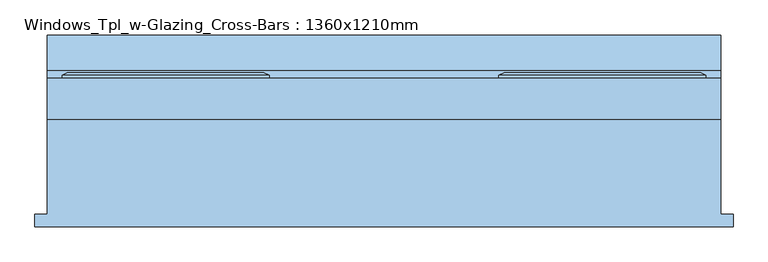
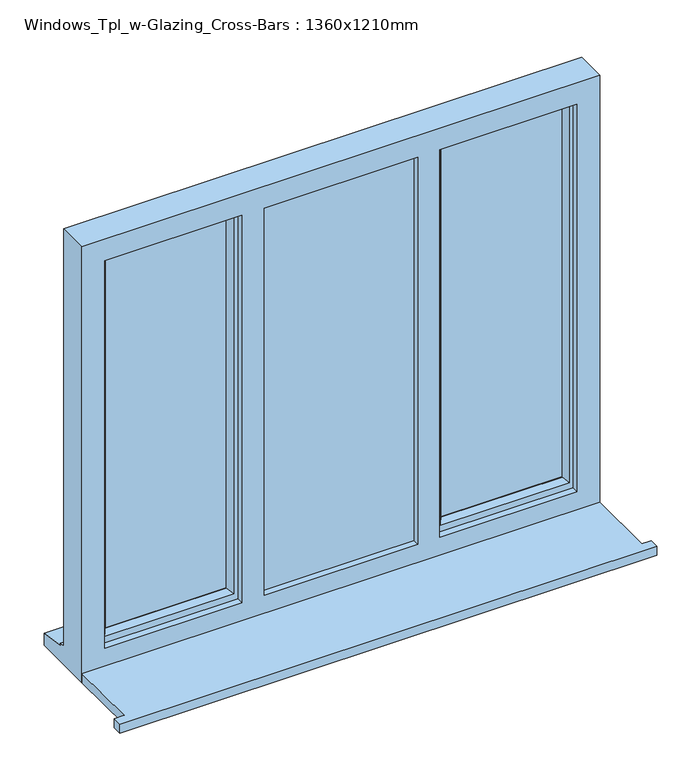
"""IFC4 building model written with IfcOpenShell, lengths in millimetres: window geometry, Windows_Tpl_w-Glazing_Cross-Bars : 1360x1210mm."""

import ifcopenshell
import ifcopenshell.guid

model = None  # the IFC model being written
_history = None  # IfcOwnerHistory: only IFC2X3 demands one
_inside = {}  # id of a spatial element -> (the spatial element, [elements in it])
_under = {}  # id of a project, library or spatial element -> (it, [spatial elements below it])
_declared = {}  # id of a project -> (the project, [libraries it declares])
_typed = {}  # id of a type object -> (the type object, [elements of that type])
_made_of = {}  # id of a material, layer set ... -> (it, [elements and type objects made of it])


def new_model(schema):
    """Start an empty IFC model of exactly this schema.

    Asked for "IFC4X3", IfcOpenShell would pick the latest addendum, in which some entities
    have other attributes; the version numbers below select the first issue.
    IFC2X3 requires an IfcOwnerHistory on every rooted entity: one is made here for all.
    """
    global model, _history
    if schema == "IFC4X3":
        model = ifcopenshell.file(schema_version=(4, 3, 0, 0))
    else:
        model = ifcopenshell.file(schema=schema)
    _inside.clear()
    _under.clear()
    _declared.clear()
    _typed.clear()
    _made_of.clear()
    _history = None
    if model.schema == "IFC2X3":
        org = make("IfcOrganization", Name="unknown")
        user = make(
            "IfcPersonAndOrganization",
            ThePerson=make("IfcPerson", FamilyName="unknown"),
            TheOrganization=org,
        )
        app = make(
            "IfcApplication",
            ApplicationDeveloper=org,
            Version="unknown",
            ApplicationFullName="unknown",
            ApplicationIdentifier="unknown",
        )
        _history = make(
            "IfcOwnerHistory",
            OwningUser=user,
            OwningApplication=app,
            ChangeAction="ADDED",
            CreationDate=0,
        )
    return model


def make(cls, **values):
    """One entity of the class cls with the attributes given. An attribute that is None is left unset."""
    return model.create_entity(
        cls, **{name: value for name, value in values.items() if value is not None}
    )


def rooted(cls, **values):
    """An entity with a GlobalId (a new one), such as an element, a storey or a relation."""
    return make(cls, GlobalId=ifcopenshell.guid.new(), OwnerHistory=_history, **values)


def si_unit(unit_type, name, prefix=None):
    """IfcSIUnit, for example si_unit("LENGTHUNIT", "METRE", prefix="MILLI")."""
    return make("IfcSIUnit", UnitType=unit_type, Prefix=prefix, Name=name)


def assignment(units):
    """IfcUnitAssignment: the units of a project."""
    return None if units is None else make("IfcUnitAssignment", Units=units)


def point(xyz):
    """IfcCartesianPoint."""
    return None if xyz is None else make("IfcCartesianPoint", Coordinates=xyz)


def direction(xyz):
    """IfcDirection."""
    return None if xyz is None else make("IfcDirection", DirectionRatios=xyz)


def frame(location, z_axis=None, x_axis=None):
    """IfcAxis2Placement3D, a coordinate frame: its origin and axes. An axis left out is left unset."""
    return make(
        "IfcAxis2Placement3D",
        Location=point(location),
        Axis=direction(z_axis),
        RefDirection=direction(x_axis),
    )


def origin():
    """The frame at (0, 0, 0) with its axes left unset."""
    return frame((0.0, 0.0, 0.0))


def place(relative_to, where):
    """IfcLocalPlacement: puts the frame where relative to a parent placement (None: the world)."""
    return make(
        "IfcLocalPlacement", PlacementRelTo=relative_to, RelativePlacement=where
    )


def context(
    kind, dimensions, precision=None, world=None, true_north=None, identifier=None
):
    """IfcGeometricRepresentationContext, for example the 3D "Model" context."""
    return make(
        "IfcGeometricRepresentationContext",
        ContextIdentifier=identifier,
        ContextType=kind,
        CoordinateSpaceDimension=dimensions,
        Precision=precision,
        WorldCoordinateSystem=world,
        TrueNorth=true_north,
    )


def project(units=None, contexts=None):
    """IfcProject with its units and contexts."""
    return rooted(
        "IfcProject",
        Name="project",
        RepresentationContexts=contexts,
        UnitsInContext=assignment(units),
    )


def spatial(cls, under=None, at=None, **own):
    """A site, building, storey or space (cls), placed at a placement, below another one or the project."""
    s = rooted(cls, ObjectPlacement=at, **own)
    if under is not None:
        _under.setdefault(under.id(), (under, []))[1].append(s)
    return s


def polyline(points):
    """IfcPolyline through the points."""
    return make("IfcPolyline", Points=[point(p) for p in points])


def outline(outer, holes=None, kind="AREA"):
    """IfcArbitraryClosedProfileDef: a profile drawn as a closed curve; with holes, ...WithVoids."""
    if holes is None:
        return make("IfcArbitraryClosedProfileDef", ProfileType=kind, OuterCurve=outer)
    return make(
        "IfcArbitraryProfileDefWithVoids",
        ProfileType=kind,
        OuterCurve=outer,
        InnerCurves=holes,
    )


def extrude(swept, where, along, depth):
    """IfcExtrudedAreaSolid: the profile swept, set in the frame where, extruded along a direction by depth."""
    return make(
        "IfcExtrudedAreaSolid",
        SweptArea=swept,
        Position=where,
        ExtrudedDirection=direction(along),
        Depth=depth,
    )


def faces_of(points, faces, orient=None, outer=None):
    """IfcFace entities. A face is a list of loops; a loop is a list of indices into points, from 0.

    orient and outer hold one flag for each loop. By default every Orientation is true, the
    first loop of a face is its IfcFaceOuterBound and the others are IfcFaceBound.
    """
    made = []
    for i, loops in enumerate(faces):
        bounds = []
        for j, loop in enumerate(loops):
            is_outer = j == 0 if outer is None else outer[i][j]
            bounds.append(
                make(
                    "IfcFaceOuterBound" if is_outer else "IfcFaceBound",
                    Bound=make("IfcPolyLoop", Polygon=[points[k] for k in loop]),
                    Orientation=True if orient is None else orient[i][j],
                )
            )
        made.append(make("IfcFace", Bounds=bounds))
    return made


def faceted_brep(points, faces, orient=None, outer=None, voids=None):
    """IfcFacetedBrep: a solid bounded by flat faces; with voids (closed shells), ...WithVoids."""
    shared = [point(p) for p in points]
    hull = make("IfcClosedShell", CfsFaces=faces_of(shared, faces, orient, outer))
    if voids is None:
        return make("IfcFacetedBrep", Outer=hull)
    return make(
        "IfcFacetedBrepWithVoids",
        Outer=hull,
        Voids=[
            make(cls, CfsFaces=faces_of(shared, fs, o, b)) for cls, fs, o, b in voids
        ],
    )


def shape(context_of_items, identifier, shape_type, items):
    """IfcShapeRepresentation: the items that make up one representation, for example the "Body"."""
    return make(
        "IfcShapeRepresentation",
        ContextOfItems=context_of_items,
        RepresentationIdentifier=identifier,
        RepresentationType=shape_type,
        Items=items,
    )


def source(mapping_origin, context_of_items, identifier, shape_type, items):
    """IfcRepresentationMap: a shape defined once, which mapped items show again and again."""
    return make(
        "IfcRepresentationMap",
        MappingOrigin=mapping_origin,
        MappedRepresentation=shape(context_of_items, identifier, shape_type, items),
    )


def transform(
    local_origin,
    x_axis=None,
    y_axis=None,
    z_axis=None,
    scale=None,
    scale2=None,
    scale3=None,
    uniform=True,
):
    """IfcCartesianTransformationOperator3D, or its non-uniform kind. x_axis, y_axis, z_axis: its Axis1, 2, 3."""
    if uniform:
        return make(
            "IfcCartesianTransformationOperator3D",
            Axis1=direction(x_axis),
            Axis2=direction(y_axis),
            LocalOrigin=point(local_origin),
            Scale=scale,
            Axis3=direction(z_axis),
        )
    return make(
        "IfcCartesianTransformationOperator3DnonUniform",
        Axis1=direction(x_axis),
        Axis2=direction(y_axis),
        LocalOrigin=point(local_origin),
        Scale=scale,
        Axis3=direction(z_axis),
        Scale2=scale2,
        Scale3=scale3,
    )


def mapped(mapping_source, mapping_target):
    """IfcMappedItem: shows the shape of a source again, moved by a transform."""
    return make(
        "IfcMappedItem", MappingSource=mapping_source, MappingTarget=mapping_target
    )


def made_of(thing, what):
    """Note that an element or type object is made of a material, layer set ...; save() writes the relation."""
    if what is not None:
        _made_of.setdefault(what.id(), (what, []))[1].append(thing)
    return thing


def element(
    cls,
    number,
    at=None,
    inside=None,
    cuts=None,
    type_object=None,
    material=None,
    context=None,
    identifier="Body",
    shape_type=None,
    held_by="IfcProductDefinitionShape",
    body=None,
    shapes=None,
    **own,
):
    """One element of the class cls, such as IfcWall. Its Tag is "e" and its number.

    at: its placement. inside: the storey or other place that contains it. cuts: it is an
    opening in that element (IfcRelVoidsElement). A single representation is given by context,
    identifier, shape_type and body (its items); several are given by shapes. held_by: the class
    of the entity that holds the representations. save() writes the other relations.
    """
    e = rooted(cls, Tag="e%d" % number, ObjectPlacement=at, **own)
    if body is not None:
        shapes = [shape(context, identifier, shape_type, body)]
    if shapes is not None:
        e.Representation = make(held_by, Representations=shapes)
    if inside is not None:
        _inside.setdefault(inside.id(), (inside, []))[1].append(e)
    if cuts is not None:
        rooted(
            "IfcRelVoidsElement", RelatingBuildingElement=cuts, RelatedOpeningElement=e
        )
    if type_object is not None:
        _typed.setdefault(type_object.id(), (type_object, []))[1].append(e)
    return made_of(e, material)


def aggregate(whole, parts):
    """IfcRelAggregates: a whole, such as a stair, and the parts it consists of."""
    return rooted("IfcRelAggregates", RelatingObject=whole, RelatedObjects=parts)


def save(model, path):
    """Write the relations noted so far, then the file.

    IfcRelAggregates (storeys below a building ...), IfcRelContainedInSpatialStructure (elements
    in a storey), IfcRelDefinesByType, IfcRelAssociatesMaterial and IfcRelDeclares: one each for
    every whole, place, type object, material and project.
    """
    for whole, parts in _under.values():
        aggregate(whole, parts)
    for where, things in _inside.values():
        rooted(
            "IfcRelContainedInSpatialStructure",
            RelatedElements=things,
            RelatingStructure=where,
        )
    for kind, things in _typed.values():
        rooted("IfcRelDefinesByType", RelatedObjects=things, RelatingType=kind)
    for what, things in _made_of.values():
        rooted("IfcRelAssociatesMaterial", RelatedObjects=things, RelatingMaterial=what)
    for by, libraries in _declared.values():
        rooted("IfcRelDeclares", RelatingContext=by, RelatedDefinitions=libraries)
    model.write(path)


def windows_tpl_w_glazing_cross_bars_1360x1210mm_fa1f7dc8(model_context):
    return source(origin(), model_context, "Body", "SolidModel", [
        extrude(outline(polyline([(-1206.6666667, -178.7934322), (-1206.6666667, -153.7934322), (-1181.6666667, -153.7934322), (-1181.6666667, 37.7065678), (178.3333333, 37.7065678), (178.3333333, -153.7934322), (203.3333333, -153.7934322), (203.3333333, -178.7934322), (-1206.6666667, -178.7934322)])), frame((0.0, 0.0, 900.0), z_axis=(0.0, 0.0, 1.0), x_axis=(1.0, 0.0, 0.0)), (0.0, 0.0, 1.0), 25.0),
        extrude(outline(polyline([(-773.3333333, 72.4565678), (-1111.6666667, 72.4565678), (-1111.6666667, 96.4565678), (-773.3333333, 96.4565678), (-773.3333333, 72.4565678)])), frame((0.0, 0.0, 993.0), z_axis=(0.0, 0.0, 1.0), x_axis=(1.0, 0.0, 0.0)), (0.0, 0.0, 1.0), 1047.0),
        extrude(outline(polyline([(108.4813711, 72.4565678), (-230.1480377, 72.4565678), (-230.1480377, 96.4565678), (108.4813711, 96.4565678), (108.4813711, 72.4565678)])), frame((0.0, 0.0, 992.8519623), z_axis=(0.0, 0.0, 1.0), x_axis=(1.0, 0.0, 0.0)), (0.0, 0.0, 1.0), 1047.2960754),
        extrude(outline(polyline([(-713.3333333, 79.7065678), (-290.0, 79.7065678), (-290.0, 55.7065678), (-713.3333333, 55.7065678), (-713.3333333, 79.7065678)])), frame((0.0, 0.0, 963.0), z_axis=(0.0, 0.0, 1.0), x_axis=(1.0, 0.0, 0.0)), (0.0, 0.0, 1.0), 1107.0),
        faceted_brep([(178.3333333, 37.7065678, 2110.0), (-1181.6666667, 37.7065678, 2110.0), (-1181.6666667, 37.7065678, 900.0), (178.3333333, 37.7065678, 900.0), (118.3333333, 37.7065678, 2050.0), (118.3333333, 37.7065678, 975.0), (-242.0, 37.7065678, 975.0), (-242.0, 37.7065678, 2050.0), (-300.0, 37.7065678, 2050.0), (-300.0, 37.7065678, 975.0), (-703.3333333, 37.7065678, 975.0), (-703.3333333, 37.7065678, 2050.0), (-761.3333333, 37.7065678, 2050.0), (-761.3333333, 37.7065678, 975.0), (-1121.6666667, 37.7065678, 975.0), (-1121.6666667, 37.7065678, 2050.0), (-1181.6666667, 120.7065678, 2110.0), (-1181.6666667, 120.7065678, 951.0), (-1181.6666667, 135.7065678, 949.68767), (-1181.6666667, 135.7065678, 944.7449676), (-1181.6666667, 208.2065678, 933.8088847), (-1181.6666667, 208.2065678, 900.0), (178.3333333, 120.7065678, 2110.0), (178.3333333, 120.7065678, 951.0), (-1141.6666667, 120.7065678, 2070.0), (-1141.6666667, 120.7065678, 963.0), (-743.3333333, 120.7065678, 963.0), (-743.3333333, 120.7065678, 2070.0), (-703.3333333, 120.7065678, 2070.0), (-703.3333333, 120.7065678, 963.0), (-300.0, 120.7065678, 963.0), (-300.0, 120.7065678, 2070.0), (-260.0, 120.7065678, 2070.0), (-260.0, 120.7065678, 963.0), (138.3333333, 120.7065678, 963.0), (138.3333333, 120.7065678, 2070.0), (-1141.6666667, 55.7065678, 2070.0), (-1141.6666667, 55.7065678, 963.0), (-713.3333333, 55.7065678, 2070.0), (-290.0, 55.7065678, 2070.0), (-290.0, 55.7065678, 963.0), (-713.3333333, 55.7065678, 963.0), (-300.0, 55.7065678, 2050.0), (-703.3333333, 55.7065678, 2050.0), (-703.3333333, 55.7065678, 975.0), (-300.0, 55.7065678, 975.0), (-260.0, 55.7065678, 2070.0), (138.3333333, 55.7065678, 2070.0), (138.3333333, 55.7065678, 963.0), (-260.0, 55.7065678, 963.0), (118.3333333, 55.7065678, 2050.0), (-242.0, 55.7065678, 2050.0), (-242.0, 55.7065678, 975.0), (118.3333333, 55.7065678, 975.0), (-743.3333333, 55.7065678, 2070.0), (-743.3333333, 55.7065678, 963.0), (-761.3333333, 55.7065678, 2050.0), (-1121.6666667, 55.7065678, 2050.0), (-1121.6666667, 55.7065678, 975.0), (-761.3333333, 55.7065678, 975.0), (-703.3333333, 79.7065678, 2070.0), (-300.0, 79.7065678, 2070.0), (-290.0, 79.7065678, 2070.0), (-713.3333333, 79.7065678, 2070.0), (178.3333333, 208.2065678, 900.0), (178.3333333, 208.2065678, 933.8088847), (178.3333333, 135.7065678, 944.7449676), (178.3333333, 135.7065678, 949.68767), (-703.3333333, 79.7065678, 963.0), (-713.3333333, 79.7065678, 963.0), (-290.0, 79.7065678, 963.0), (-300.0, 79.7065678, 963.0)], [[[0, 1, 2, 3], [4, 5, 6, 7], [8, 9, 10, 11], [12, 13, 14, 15]], [[2, 1, 16, 17, 18, 19, 20, 21]], [[17, 16, 22, 23], [24, 25, 26, 27], [28, 29, 30, 31], [32, 33, 34, 35]], [[25, 24, 36, 37]], [[38, 39, 40, 41], [42, 43, 44, 45]], [[46, 47, 48, 49], [50, 51, 52, 53]], [[36, 54, 55, 37], [56, 57, 58, 59]], [[57, 15, 14, 58]], [[1, 0, 22, 16]], [[36, 24, 27, 54]], [[35, 47, 46, 32]], [[60, 28, 31, 61, 62, 39, 38, 63]], [[15, 57, 56, 12]], [[50, 4, 7, 51]], [[11, 43, 42, 8]], [[23, 22, 0, 3, 64, 65, 66, 67]], [[35, 34, 48, 47]], [[4, 50, 53, 5]], [[43, 11, 10, 44]], [[12, 56, 59, 13]], [[27, 26, 55, 54]], [[29, 28, 60, 68]], [[68, 60, 63, 69]], [[69, 63, 38, 41]], [[62, 70, 40, 39]], [[70, 62, 61, 71]], [[71, 61, 31, 30]], [[33, 32, 46, 49]], [[51, 7, 6, 52]], [[8, 42, 45, 9]], [[64, 3, 2, 21]], [[65, 64, 21, 20]], [[66, 65, 20, 19]], [[67, 66, 19, 18]], [[23, 67, 18, 17]], [[26, 25, 37, 55]], [[34, 33, 49, 48]], [[41, 40, 70, 71, 30, 29, 68, 69]], [[6, 5, 53, 52]], [[45, 44, 10, 9]], [[59, 58, 14, 13]]]),
        extrude(outline(polyline([(963.0, -511.6666667), (963.0, -491.6666667), (1506.5, -491.6666667), (1506.5, -290.0), (1526.5, -290.0), (1526.5, -491.6666667), (2070.0, -491.6666667), (2070.0, -511.6666667), (1526.5, -511.6666667), (1526.5, -713.3333333), (1506.5, -713.3333333), (1506.5, -511.6666667), (963.0, -511.6666667)])), frame((0.0, 63.7065678, 0.0), z_axis=(0.0, 1.0, 0.0), x_axis=(0.0, 0.0, 1.0)), (0.0, 0.0, 1.0), 8.0),
        extrude(outline(polyline([(993.0, -70.8333333), (993.0, -50.8333333), (1506.5, -50.8333333), (1506.5, 108.3333333), (1526.5, 108.3333333), (1526.5, -50.8333333), (2040.1480377, -50.8333333), (2040.1480377, -70.8333333), (1526.5, -70.8333333), (1526.5, -230.1480377), (1506.5, -230.1480377), (1506.5, -70.8333333), (993.0, -70.8333333)])), frame((0.0, 92.7065678, 0.0), z_axis=(0.0, 1.0, 0.0), x_axis=(0.0, 0.0, 1.0)), (0.0, 0.0, 1.0), 8.0),
        extrude(outline(polyline([(993.0, -952.5), (993.0, -932.5), (1506.5, -932.5), (1506.5, -773.3333333), (1526.5, -773.3333333), (1526.5, -932.5), (2040.1480377, -932.5), (2040.1480377, -952.5), (1526.5, -952.5), (1526.5, -1111.6666667), (1506.5, -1111.6666667), (1506.5, -952.5), (993.0, -952.5)])), frame((0.0, 92.7065678, 0.0), z_axis=(0.0, 1.0, 0.0), x_axis=(0.0, 0.0, 1.0)), (0.0, 0.0, 1.0), 8.0),
        faceted_brep([(-733.3333333, 120.7065678, 2080.0), (-733.3333333, 126.4800705, 2080.0), (-1151.6666667, 126.4800705, 2080.0), (-1151.6666667, 120.7065678, 2080.0), (-743.3333333, 55.7065678, 2070.0), (-743.3333333, 120.7065678, 2070.0), (-1141.6666667, 120.7065678, 2070.0), (-1141.6666667, 55.7065678, 2070.0), (-783.3333333, 70.1994677, 2030.0), (-773.1852956, 55.7065678, 2040.1480377), (-1111.8147044, 55.7065678, 2040.1480377), (-1101.6666667, 70.1994677, 2030.0), (-783.3333333, 84.7065678, 2030.0), (-1101.6666667, 84.7065678, 2030.0), (-773.3333333, 108.7065678, 2040.0), (-773.3333333, 84.7065678, 2040.0), (-1111.6666667, 84.7065678, 2040.0), (-1111.6666667, 108.7065678, 2040.0), (-783.3333333, 126.4800705, 2030.0), (-783.3333333, 108.7065678, 2030.0), (-1101.6666667, 108.7065678, 2030.0), (-1101.6666667, 126.4800705, 2030.0), (-765.8875785, 132.2535732, 2047.4457548), (-1119.1124215, 132.2535732, 2047.4457548), (-744.117943, 132.2535732, 2069.2153903), (-1140.882057, 132.2535732, 2069.2153903), (-1151.6666667, 126.4800705, 953.0), (-1151.6666667, 120.7065678, 953.0), (-1141.6666667, 120.7065678, 963.0), (-1141.6666667, 55.7065678, 963.0), (-1111.8147044, 55.7065678, 992.8519623), (-1101.6666667, 70.1994677, 1003.0), (-1101.6666667, 84.7065678, 1003.0), (-1111.6666667, 84.7065678, 993.0), (-1111.6666667, 108.7065678, 993.0), (-1101.6666667, 108.7065678, 1003.0), (-1101.6666667, 126.4800705, 1003.0), (-1119.1124215, 132.2535732, 985.5542452), (-1140.882057, 132.2535732, 963.7846097), (-733.3333333, 126.4800705, 953.0), (-733.3333333, 120.7065678, 953.0), (-743.3333333, 120.7065678, 963.0), (-743.3333333, 55.7065678, 963.0), (-773.1852956, 55.7065678, 992.8519623), (-783.3333333, 70.1994677, 1003.0), (-783.3333333, 84.7065678, 1003.0), (-773.3333333, 84.7065678, 993.0), (-773.3333333, 108.7065678, 993.0), (-783.3333333, 108.7065678, 1003.0), (-783.3333333, 126.4800705, 1003.0), (-765.8875785, 132.2535732, 985.5542452), (-744.117943, 132.2535732, 963.7846097)], [[[0, 1, 2, 3]], [[4, 5, 6, 7]], [[8, 9, 10, 11]], [[12, 8, 11, 13]], [[14, 15, 16, 17]], [[18, 19, 20, 21]], [[22, 18, 21, 23]], [[1, 24, 25, 2]], [[3, 2, 26, 27]], [[7, 6, 28, 29]], [[11, 10, 30, 31]], [[13, 11, 31, 32]], [[17, 16, 33, 34]], [[21, 20, 35, 36]], [[23, 21, 36, 37]], [[2, 25, 38, 26]], [[27, 26, 39, 40]], [[0, 3, 27, 40], [41, 28, 6, 5]], [[29, 28, 41, 42]], [[4, 7, 29, 42], [43, 30, 10, 9]], [[31, 30, 43, 44]], [[32, 31, 44, 45]], [[46, 33, 16, 15], [12, 13, 32, 45]], [[34, 33, 46, 47]], [[14, 17, 34, 47], [48, 35, 20, 19]], [[36, 35, 48, 49]], [[37, 36, 49, 50]], [[51, 38, 25, 24], [22, 23, 37, 50]], [[26, 38, 51, 39]], [[40, 39, 1, 0]], [[42, 41, 5, 4]], [[44, 43, 9, 8]], [[45, 44, 8, 12]], [[47, 46, 15, 14]], [[49, 48, 19, 18]], [[50, 49, 18, 22]], [[39, 51, 24, 1]]]),
        faceted_brep([(-270.0, 120.7065678, 2080.0), (-270.0, 126.4800705, 2080.0), (-270.0, 126.4800705, 953.0), (-270.0, 120.7065678, 953.0), (-260.0, 55.7065678, 2070.0), (-260.0, 120.7065678, 2070.0), (-260.0, 120.7065678, 963.0), (-260.0, 55.7065678, 963.0), (-220.0, 70.1994677, 2030.0), (-230.1480377, 55.7065678, 2040.1480377), (-230.1480377, 55.7065678, 992.8519623), (-220.0, 70.1994677, 1003.0), (-220.0, 84.7065678, 2030.0), (-220.0, 84.7065678, 1003.0), (-230.0, 108.7065678, 2040.0), (-230.0, 84.7065678, 2040.0), (-230.0, 84.7065678, 993.0), (-230.0, 108.7065678, 993.0), (-220.0, 126.4800705, 2030.0), (-220.0, 108.7065678, 2030.0), (-220.0, 108.7065678, 1003.0), (-220.0, 126.4800705, 1003.0), (-237.4457548, 132.2535732, 2047.4457548), (-237.4457548, 132.2535732, 985.5542452), (-259.2153903, 132.2535732, 2069.2153903), (-259.2153903, 132.2535732, 963.7846097), (148.3333333, 126.4800705, 953.0), (148.3333333, 120.7065678, 953.0), (138.3333333, 120.7065678, 963.0), (138.3333333, 55.7065678, 963.0), (108.4813711, 55.7065678, 992.8519623), (98.3333333, 70.1994677, 1003.0), (98.3333333, 84.7065678, 1003.0), (108.3333333, 84.7065678, 993.0), (108.3333333, 108.7065678, 993.0), (98.3333333, 108.7065678, 1003.0), (98.3333333, 126.4800705, 1003.0), (115.7790881, 132.2535732, 985.5542452), (137.5487236, 132.2535732, 963.7846097), (148.3333333, 126.4800705, 2080.0), (148.3333333, 120.7065678, 2080.0), (138.3333333, 120.7065678, 2070.0), (138.3333333, 55.7065678, 2070.0), (108.4813711, 55.7065678, 2040.1480377), (98.3333333, 70.1994677, 2030.0), (98.3333333, 84.7065678, 2030.0), (108.3333333, 84.7065678, 2040.0), (108.3333333, 108.7065678, 2040.0), (98.3333333, 108.7065678, 2030.0), (98.3333333, 126.4800705, 2030.0), (115.7790881, 132.2535732, 2047.4457548), (137.5487236, 132.2535732, 2069.2153903)], [[[0, 1, 2, 3]], [[4, 5, 6, 7]], [[8, 9, 10, 11]], [[12, 8, 11, 13]], [[14, 15, 16, 17]], [[18, 19, 20, 21]], [[22, 18, 21, 23]], [[1, 24, 25, 2]], [[3, 2, 26, 27]], [[7, 6, 28, 29]], [[11, 10, 30, 31]], [[13, 11, 31, 32]], [[17, 16, 33, 34]], [[21, 20, 35, 36]], [[23, 21, 36, 37]], [[2, 25, 38, 26]], [[27, 26, 39, 40]], [[29, 28, 41, 42]], [[31, 30, 43, 44]], [[32, 31, 44, 45]], [[34, 33, 46, 47]], [[36, 35, 48, 49]], [[37, 36, 49, 50]], [[26, 38, 51, 39]], [[40, 39, 1, 0]], [[3, 27, 40, 0], [5, 41, 28, 6]], [[42, 41, 5, 4]], [[7, 29, 42, 4], [9, 43, 30, 10]], [[44, 43, 9, 8]], [[45, 44, 8, 12]], [[15, 46, 33, 16], [13, 32, 45, 12]], [[47, 46, 15, 14]], [[17, 34, 47, 14], [19, 48, 35, 20]], [[49, 48, 19, 18]], [[50, 49, 18, 22]], [[24, 51, 38, 25], [23, 37, 50, 22]], [[39, 51, 24, 1]]]),
    ])


if __name__ == "__main__":
    model = new_model("IFC4")
    model_context = context("Model", 3, world=origin())
    ifc_project = project(units=[si_unit("LENGTHUNIT", "METRE", prefix="MILLI")], contexts=[model_context])
    site = spatial("IfcSite", under=ifc_project)
    building = spatial("IfcBuilding", under=site)
    placement = place(None, origin())
    windows_tpl_w_glazing_cross_bars_1360x1210mm_shape = windows_tpl_w_glazing_cross_bars_1360x1210mm_fa1f7dc8(model_context)
    element("IfcWindow", 1, ObjectType="Windows_Tpl_w-Glazing_Cross-Bars : 1360x1210mm", at=placement, inside=building, context=model_context, shape_type="MappedRepresentation", body=[
        mapped(windows_tpl_w_glazing_cross_bars_1360x1210mm_shape, transform((0.0, 0.0, 0.0), x_axis=(1.0, 0.0, 0.0), y_axis=(0.0, 1.0, 0.0), z_axis=(0.0, 0.0, 1.0))),
    ])
    save(model, "model.ifc")

# Revit data of these elements
# Project information
#   Project Issue Date = "Issue Date"
#   Project Status = "Project Status"
#   Client Name = "Owner"
#   Project Address = "Enter address here"
#   Project Name = "Project Management Assignment 1"
#   Project Number = "PMBM01"
# Type "Windows_Tpl_w-Glazing_Cross-Bars : 1360x1210mm"
#   Type Mark = "53"
#   Operation = "TriplePanelVertical"
#   Construction Type Id = "GSP4R"
#   Manufacturer = "Revit"
#   Keynote = "L10"
#   Analytic Construction = "1/8 in Pilkington single glazing"
#   Wrap Layers (Ext) from Ext = 102.5 mm
#   Wrap Layers (Int) from Ext = 177.5 mm
#   Window Board Projection = 25 mm
#   Window Board Extension = 25 mm
#   Visual Light Transmittance = 0.9
#   Solar Heat Gain Coefficient = 0.78
#   Rough Width = 1360 mm
#   Rough Height = 1210 mm
#   Height = 1210 mm
#   Width = 1360 mm
#   Heat Transfer Coefficient (U) = 3.6886 W/(m²·K)
#   Glazing Thickness = 24 mm
#   Glazing Bar Thickness = 20 mm
#   FrameOffset - External = 50 mm
#   Frame Depth = 65 mm
#   Default Head Height = 2110 mm
#   Cill Depth = 87.5 mm
#   Cavity Closer Width = 50 mm
#   Cavity Closer Offset from Ext = 102.5 mm
#   Cavity Closer Depth = 85 mm
#   Vis - Glazing Bars = yes
#   Vis - Cavity Closers = yes
#   Define Thermal Properties by = 1
#   Material Trim = Window Frame
#   Material Glazing Bars = Window Frame
#   Material Glass = Glass
#   Material Frame = Window Frame
#   Wall Closure = (empty or 0)
# Element 1 (IfcWindow, "Windows_Tpl_w-Glazing_Cross-Bars : 1360x1210mm")
#   Materials on its faces: "Window Frame", "Glass"
# Materials
#   "Window Frame": class "Miscellaneous", colour RGB 249 249 249, transparency 0, Keynote = "L10"
#   "Glass": class "Glass", colour RGB 0 128 192, transparency 0.9, Description = "Soda Lime Glass", Cost = 0
